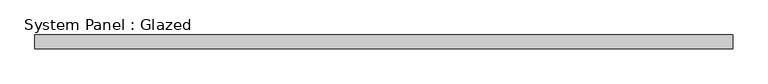
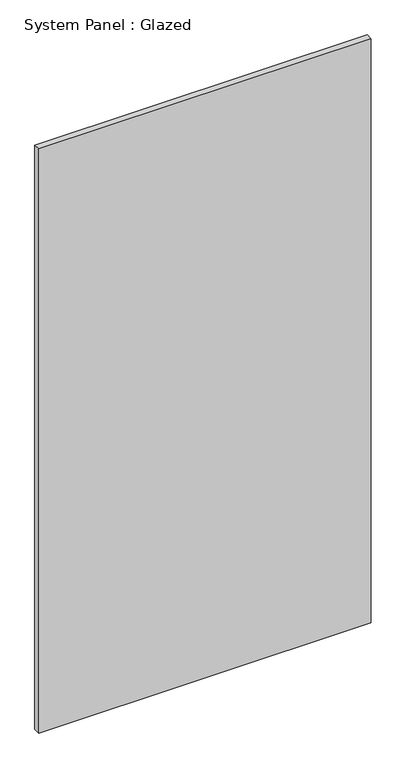
"""IFC4 building model written with IfcOpenShell, lengths in millimetres: plate geometry, System Panel : Glazed."""

import ifcopenshell
import ifcopenshell.guid

model = None  # the IFC model being written
_history = None  # IfcOwnerHistory: only IFC2X3 demands one
_inside = {}  # id of a spatial element -> (the spatial element, [elements in it])
_under = {}  # id of a project, library or spatial element -> (it, [spatial elements below it])
_declared = {}  # id of a project -> (the project, [libraries it declares])
_typed = {}  # id of a type object -> (the type object, [elements of that type])
_made_of = {}  # id of a material, layer set ... -> (it, [elements and type objects made of it])


def new_model(schema):
    """Start an empty IFC model of exactly this schema.

    Asked for "IFC4X3", IfcOpenShell would pick the latest addendum, in which some entities
    have other attributes; the version numbers below select the first issue.
    IFC2X3 requires an IfcOwnerHistory on every rooted entity: one is made here for all.
    """
    global model, _history
    if schema == "IFC4X3":
        model = ifcopenshell.file(schema_version=(4, 3, 0, 0))
    else:
        model = ifcopenshell.file(schema=schema)
    _inside.clear()
    _under.clear()
    _declared.clear()
    _typed.clear()
    _made_of.clear()
    _history = None
    if model.schema == "IFC2X3":
        org = make("IfcOrganization", Name="unknown")
        user = make(
            "IfcPersonAndOrganization",
            ThePerson=make("IfcPerson", FamilyName="unknown"),
            TheOrganization=org,
        )
        app = make(
            "IfcApplication",
            ApplicationDeveloper=org,
            Version="unknown",
            ApplicationFullName="unknown",
            ApplicationIdentifier="unknown",
        )
        _history = make(
            "IfcOwnerHistory",
            OwningUser=user,
            OwningApplication=app,
            ChangeAction="ADDED",
            CreationDate=0,
        )
    return model


def make(cls, **values):
    """One entity of the class cls with the attributes given. An attribute that is None is left unset."""
    return model.create_entity(
        cls, **{name: value for name, value in values.items() if value is not None}
    )


def rooted(cls, **values):
    """An entity with a GlobalId (a new one), such as an element, a storey or a relation."""
    return make(cls, GlobalId=ifcopenshell.guid.new(), OwnerHistory=_history, **values)


def si_unit(unit_type, name, prefix=None):
    """IfcSIUnit, for example si_unit("LENGTHUNIT", "METRE", prefix="MILLI")."""
    return make("IfcSIUnit", UnitType=unit_type, Prefix=prefix, Name=name)


def assignment(units):
    """IfcUnitAssignment: the units of a project."""
    return None if units is None else make("IfcUnitAssignment", Units=units)


def point(xyz):
    """IfcCartesianPoint."""
    return None if xyz is None else make("IfcCartesianPoint", Coordinates=xyz)


def direction(xyz):
    """IfcDirection."""
    return None if xyz is None else make("IfcDirection", DirectionRatios=xyz)


def frame(location, z_axis=None, x_axis=None):
    """IfcAxis2Placement3D, a coordinate frame: its origin and axes. An axis left out is left unset."""
    return make(
        "IfcAxis2Placement3D",
        Location=point(location),
        Axis=direction(z_axis),
        RefDirection=direction(x_axis),
    )


def origin():
    """The frame at (0, 0, 0) with its axes left unset."""
    return frame((0.0, 0.0, 0.0))


def origin_with_axes():
    """The frame at (0, 0, 0) with the z axis (0, 0, 1) and the x axis (1, 0, 0) written out."""
    return frame((0.0, 0.0, 0.0), z_axis=(0.0, 0.0, 1.0), x_axis=(1.0, 0.0, 0.0))


def place(relative_to, where):
    """IfcLocalPlacement: puts the frame where relative to a parent placement (None: the world)."""
    return make(
        "IfcLocalPlacement", PlacementRelTo=relative_to, RelativePlacement=where
    )


def context(
    kind, dimensions, precision=None, world=None, true_north=None, identifier=None
):
    """IfcGeometricRepresentationContext, for example the 3D "Model" context."""
    return make(
        "IfcGeometricRepresentationContext",
        ContextIdentifier=identifier,
        ContextType=kind,
        CoordinateSpaceDimension=dimensions,
        Precision=precision,
        WorldCoordinateSystem=world,
        TrueNorth=true_north,
    )


def project(units=None, contexts=None):
    """IfcProject with its units and contexts."""
    return rooted(
        "IfcProject",
        Name="project",
        RepresentationContexts=contexts,
        UnitsInContext=assignment(units),
    )


def spatial(cls, under=None, at=None, **own):
    """A site, building, storey or space (cls), placed at a placement, below another one or the project."""
    s = rooted(cls, ObjectPlacement=at, **own)
    if under is not None:
        _under.setdefault(under.id(), (under, []))[1].append(s)
    return s


def polyline(points):
    """IfcPolyline through the points."""
    return make("IfcPolyline", Points=[point(p) for p in points])


def outline(outer, holes=None, kind="AREA"):
    """IfcArbitraryClosedProfileDef: a profile drawn as a closed curve; with holes, ...WithVoids."""
    if holes is None:
        return make("IfcArbitraryClosedProfileDef", ProfileType=kind, OuterCurve=outer)
    return make(
        "IfcArbitraryProfileDefWithVoids",
        ProfileType=kind,
        OuterCurve=outer,
        InnerCurves=holes,
    )


def extrude(swept, where, along, depth):
    """IfcExtrudedAreaSolid: the profile swept, set in the frame where, extruded along a direction by depth."""
    return make(
        "IfcExtrudedAreaSolid",
        SweptArea=swept,
        Position=where,
        ExtrudedDirection=direction(along),
        Depth=depth,
    )


def shape(context_of_items, identifier, shape_type, items):
    """IfcShapeRepresentation: the items that make up one representation, for example the "Body"."""
    return make(
        "IfcShapeRepresentation",
        ContextOfItems=context_of_items,
        RepresentationIdentifier=identifier,
        RepresentationType=shape_type,
        Items=items,
    )


def source(mapping_origin, context_of_items, identifier, shape_type, items):
    """IfcRepresentationMap: a shape defined once, which mapped items show again and again."""
    return make(
        "IfcRepresentationMap",
        MappingOrigin=mapping_origin,
        MappedRepresentation=shape(context_of_items, identifier, shape_type, items),
    )


def transform(
    local_origin,
    x_axis=None,
    y_axis=None,
    z_axis=None,
    scale=None,
    scale2=None,
    scale3=None,
    uniform=True,
):
    """IfcCartesianTransformationOperator3D, or its non-uniform kind. x_axis, y_axis, z_axis: its Axis1, 2, 3."""
    if uniform:
        return make(
            "IfcCartesianTransformationOperator3D",
            Axis1=direction(x_axis),
            Axis2=direction(y_axis),
            LocalOrigin=point(local_origin),
            Scale=scale,
            Axis3=direction(z_axis),
        )
    return make(
        "IfcCartesianTransformationOperator3DnonUniform",
        Axis1=direction(x_axis),
        Axis2=direction(y_axis),
        LocalOrigin=point(local_origin),
        Scale=scale,
        Axis3=direction(z_axis),
        Scale2=scale2,
        Scale3=scale3,
    )


def mapped(mapping_source, mapping_target):
    """IfcMappedItem: shows the shape of a source again, moved by a transform."""
    return make(
        "IfcMappedItem", MappingSource=mapping_source, MappingTarget=mapping_target
    )


def made_of(thing, what):
    """Note that an element or type object is made of a material, layer set ...; save() writes the relation."""
    if what is not None:
        _made_of.setdefault(what.id(), (what, []))[1].append(thing)
    return thing


def element(
    cls,
    number,
    at=None,
    inside=None,
    cuts=None,
    type_object=None,
    material=None,
    context=None,
    identifier="Body",
    shape_type=None,
    held_by="IfcProductDefinitionShape",
    body=None,
    shapes=None,
    **own,
):
    """One element of the class cls, such as IfcWall. Its Tag is "e" and its number.

    at: its placement. inside: the storey or other place that contains it. cuts: it is an
    opening in that element (IfcRelVoidsElement). A single representation is given by context,
    identifier, shape_type and body (its items); several are given by shapes. held_by: the class
    of the entity that holds the representations. save() writes the other relations.
    """
    e = rooted(cls, Tag="e%d" % number, ObjectPlacement=at, **own)
    if body is not None:
        shapes = [shape(context, identifier, shape_type, body)]
    if shapes is not None:
        e.Representation = make(held_by, Representations=shapes)
    if inside is not None:
        _inside.setdefault(inside.id(), (inside, []))[1].append(e)
    if cuts is not None:
        rooted(
            "IfcRelVoidsElement", RelatingBuildingElement=cuts, RelatedOpeningElement=e
        )
    if type_object is not None:
        _typed.setdefault(type_object.id(), (type_object, []))[1].append(e)
    return made_of(e, material)


def aggregate(whole, parts):
    """IfcRelAggregates: a whole, such as a stair, and the parts it consists of."""
    return rooted("IfcRelAggregates", RelatingObject=whole, RelatedObjects=parts)


def save(model, path):
    """Write the relations noted so far, then the file.

    IfcRelAggregates (storeys below a building ...), IfcRelContainedInSpatialStructure (elements
    in a storey), IfcRelDefinesByType, IfcRelAssociatesMaterial and IfcRelDeclares: one each for
    every whole, place, type object, material and project.
    """
    for whole, parts in _under.values():
        aggregate(whole, parts)
    for where, things in _inside.values():
        rooted(
            "IfcRelContainedInSpatialStructure",
            RelatedElements=things,
            RelatingStructure=where,
        )
    for kind, things in _typed.values():
        rooted("IfcRelDefinesByType", RelatedObjects=things, RelatingType=kind)
    for what, things in _made_of.values():
        rooted("IfcRelAssociatesMaterial", RelatedObjects=things, RelatingMaterial=what)
    for by, libraries in _declared.values():
        rooted("IfcRelDeclares", RelatingContext=by, RelatedDefinitions=libraries)
    model.write(path)


def system_panel_glazed_a88fc5f3(model_context):
    return source(origin(), model_context, "Body", "SweptSolid", [
        extrude(outline(polyline([(633.0541355, 24.5), (-633.0541355, 24.5), (-633.0541355, 49.5), (633.0541355, 49.5), (633.0541355, 24.5)])), origin_with_axes(), (0.0, 0.0, 1.0), 2350.0),
    ])


if __name__ == "__main__":
    model = new_model("IFC4")
    model_context = context("Model", 3, world=origin())
    ifc_project = project(units=[si_unit("LENGTHUNIT", "METRE", prefix="MILLI")], contexts=[model_context])
    site = spatial("IfcSite", under=ifc_project)
    building = spatial("IfcBuilding", under=site)
    placement = place(None, origin())
    system_panel_glazed_shape = system_panel_glazed_a88fc5f3(model_context)
    element("IfcPlate", 1, ObjectType="System Panel : Glazed", at=placement, inside=building, context=model_context, shape_type="MappedRepresentation", body=[
        mapped(system_panel_glazed_shape, transform((0.0, 0.0, 0.0), x_axis=(1.0, 0.0, 0.0), y_axis=(0.0, 1.0, 0.0), z_axis=(0.0, 0.0, 1.0))),
    ])
    save(model, "model.ifc")

# Revit data of these elements
# Type "System Panel : Glazed"
#   Construction Type Id = "GSP4R"
#   Analytic Construction = "1/8 in Pilkington single glazing"
#   Visual Light Transmittance = 0.9
#   Solar Heat Gain Coefficient = 0.86
#   Heat Transfer Coefficient (U) = 6.7069 W/(m²·K)
#   Define Thermal Properties by = 1
# Element 1 (IfcPlate, "System Panel : Glazed")
#   Materials on its faces: "Glass"
# Materials
#   "Glass": class "Glass", colour RGB 0 128 192, transparency 0.9, Description = "Soda Lime Glass", Cost = 0
